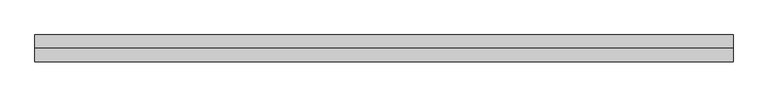
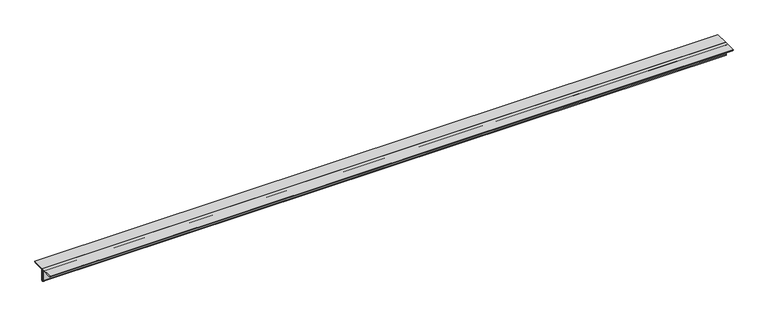
"""IFC4 building model written with IfcOpenShell, lengths in millimetres: member geometry, Steel Framing_2Ls_KS : H_SB_AR_S02_2Ls-100x100x10_VBR1."""

from ifc_helpers import new_model, si_unit, point, frame, frame_2d, origin, place, context, project, spatial, polyline, circle_curve, trimmed, segment, composite_curve, outline, extrude, source, transform, mapped, element, save


def member_ae933dc9(model_context):
    return source(origin(), model_context, "Body", "SweptSolid", [
        extrude(outline(composite_curve([segment(polyline([(0.0, 28.2), (0.0, -71.8)]), True, "CONTINUOUS"), segment(trimmed(circle_curve(frame_2d((0.0, -61.8)), 10.0), [point((0.0, -71.8))], [point((-10.0, -61.8))], False, "CARTESIAN"), True, "CONTINUOUS"), segment(polyline([(-10.0, -61.8), (-10.0, 8.2)]), True, "CONTINUOUS"), segment(trimmed(circle_curve(frame_2d((-20.0, 8.2)), 10.0), [point((-10.0, 8.2))], [point((-20.0, 18.2))], True, "CARTESIAN"), True, "CONTINUOUS"), segment(polyline([(-20.0, 18.2), (-90.0, 18.2)]), True, "CONTINUOUS"), segment(trimmed(circle_curve(frame_2d((-90.0, 28.2)), 10.0), [point((-90.0, 18.2))], [point((-100.0, 28.2))], False, "CARTESIAN"), True, "CONTINUOUS"), segment(polyline([(-100.0, 28.2), (0.0, 28.2)]), True, "CONTINUOUS")], self_intersect=False)), frame((-2590.3354834, 0.0, 0.0), z_axis=(1.0, 0.0, 0.0), x_axis=(0.0, 1.0, 0.0)), (0.0, 0.0, 1.0), 5195.0614478),
        extrude(outline(composite_curve([segment(polyline([(0.0, 28.2), (100.0, 28.2)]), True, "CONTINUOUS"), segment(trimmed(circle_curve(frame_2d((90.0, 28.2)), 10.0), [point((100.0, 28.2))], [point((90.0, 18.2))], False, "CARTESIAN"), True, "CONTINUOUS"), segment(polyline([(90.0, 18.2), (20.0, 18.2)]), True, "CONTINUOUS"), segment(trimmed(circle_curve(frame_2d((20.0, 8.2)), 10.0), [point((20.0, 18.2))], [point((10.0, 8.2))], True, "CARTESIAN"), True, "CONTINUOUS"), segment(polyline([(10.0, 8.2), (10.0, -61.8)]), True, "CONTINUOUS"), segment(trimmed(circle_curve(frame_2d((0.0, -61.8)), 10.0), [point((10.0, -61.8))], [point((0.0, -71.8))], False, "CARTESIAN"), True, "CONTINUOUS"), segment(polyline([(0.0, -71.8), (0.0, 28.2)]), True, "CONTINUOUS")], self_intersect=False)), frame((-2590.3354834, 0.0, 0.0), z_axis=(1.0, 0.0, 0.0), x_axis=(0.0, 1.0, 0.0)), (0.0, 0.0, 1.0), 5195.0614478),
    ])


if __name__ == "__main__":
    model = new_model("IFC4")
    model_context = context("Model", 3, world=origin())
    ifc_project = project(units=[si_unit("LENGTHUNIT", "METRE", prefix="MILLI")], contexts=[model_context])
    site = spatial("IfcSite", under=ifc_project)
    building = spatial("IfcBuilding", under=site)
    placement = place(None, origin())
    member_shape = member_ae933dc9(model_context)
    element("IfcMember", 1, ObjectType="Steel Framing_2Ls_KS : H_SB_AR_S02_2Ls-100x100x10_VBR1", at=placement, inside=building, context=model_context, shape_type="MappedRepresentation", body=[
        mapped(member_shape, transform((0.0, 0.0, 0.0), x_axis=(1.0, 0.0, 0.0), y_axis=(0.0, 1.0, 0.0), z_axis=(0.0, 0.0, 1.0))),
    ])
    save(model, "model.ifc")

# Revit data of these elements
# Type "Steel Framing_2Ls_KS : H_SB_AR_S02_2Ls-100x100x10_VBR1"
#   Type Comments = "MAIN"
#   Type Mark = "VBR1"
#   H_SectionID = "2Ls-100x100x10"
#   Assembly Code = "B10"
#   Legs = "LLBB"
#   H_Ratio for Additional Steel Plate = 0.2
#   W = 0
#   Perimeter = 0.80 m²/m
#   Nominal Weight = 29.80 kgf/m
#   Length [instance default] = 1524 mm
#   Space = 0 mm
#   b = 100 mm
#   d = 100 mm
#   t = 10 mm
#   y = 28.2 mm
#   A = 0.0038 m²
#   Structural Material [instance default] = Steel, 45-345
# Element 1 (IfcMember, "Steel Framing_2Ls_KS : H_SB_AR_S02_2Ls-100x100x10_VBR1")
#   Materials on its faces: "Steel, 45-345"
# Materials
#   "Steel, 45-345": class "Metal", colour RGB 189 187 185, transparency 0, Description = "Steel 345 MPa", Cost = 0
